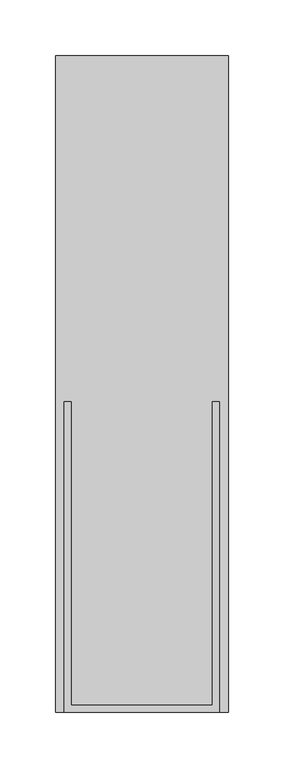
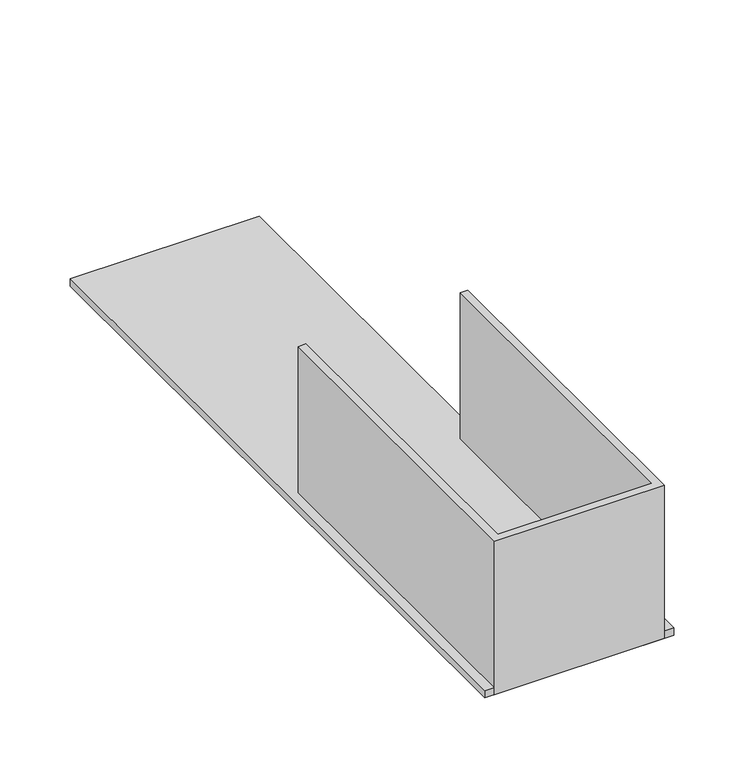
"""IFC4 building model written with IfcOpenShell, lengths in millimetres: fastener geometry, SIMPSON -THGBV - Truss Girder Hanger : SIMPSON -THGBV5.50/11 - HDG."""

import ifcopenshell
import ifcopenshell.guid

model = None  # the IFC model being written
_history = None  # IfcOwnerHistory: only IFC2X3 demands one
_inside = {}  # id of a spatial element -> (the spatial element, [elements in it])
_under = {}  # id of a project, library or spatial element -> (it, [spatial elements below it])
_declared = {}  # id of a project -> (the project, [libraries it declares])
_typed = {}  # id of a type object -> (the type object, [elements of that type])
_made_of = {}  # id of a material, layer set ... -> (it, [elements and type objects made of it])


def new_model(schema):
    """Start an empty IFC model of exactly this schema.

    Asked for "IFC4X3", IfcOpenShell would pick the latest addendum, in which some entities
    have other attributes; the version numbers below select the first issue.
    IFC2X3 requires an IfcOwnerHistory on every rooted entity: one is made here for all.
    """
    global model, _history
    if schema == "IFC4X3":
        model = ifcopenshell.file(schema_version=(4, 3, 0, 0))
    else:
        model = ifcopenshell.file(schema=schema)
    _inside.clear()
    _under.clear()
    _declared.clear()
    _typed.clear()
    _made_of.clear()
    _history = None
    if model.schema == "IFC2X3":
        org = make("IfcOrganization", Name="unknown")
        user = make(
            "IfcPersonAndOrganization",
            ThePerson=make("IfcPerson", FamilyName="unknown"),
            TheOrganization=org,
        )
        app = make(
            "IfcApplication",
            ApplicationDeveloper=org,
            Version="unknown",
            ApplicationFullName="unknown",
            ApplicationIdentifier="unknown",
        )
        _history = make(
            "IfcOwnerHistory",
            OwningUser=user,
            OwningApplication=app,
            ChangeAction="ADDED",
            CreationDate=0,
        )
    return model


def make(cls, **values):
    """One entity of the class cls with the attributes given. An attribute that is None is left unset."""
    return model.create_entity(
        cls, **{name: value for name, value in values.items() if value is not None}
    )


def rooted(cls, **values):
    """An entity with a GlobalId (a new one), such as an element, a storey or a relation."""
    return make(cls, GlobalId=ifcopenshell.guid.new(), OwnerHistory=_history, **values)


def si_unit(unit_type, name, prefix=None):
    """IfcSIUnit, for example si_unit("LENGTHUNIT", "METRE", prefix="MILLI")."""
    return make("IfcSIUnit", UnitType=unit_type, Prefix=prefix, Name=name)


def assignment(units):
    """IfcUnitAssignment: the units of a project."""
    return None if units is None else make("IfcUnitAssignment", Units=units)


def point(xyz):
    """IfcCartesianPoint."""
    return None if xyz is None else make("IfcCartesianPoint", Coordinates=xyz)


def direction(xyz):
    """IfcDirection."""
    return None if xyz is None else make("IfcDirection", DirectionRatios=xyz)


def frame(location, z_axis=None, x_axis=None):
    """IfcAxis2Placement3D, a coordinate frame: its origin and axes. An axis left out is left unset."""
    return make(
        "IfcAxis2Placement3D",
        Location=point(location),
        Axis=direction(z_axis),
        RefDirection=direction(x_axis),
    )


def origin():
    """The frame at (0, 0, 0) with its axes left unset."""
    return frame((0.0, 0.0, 0.0))


def origin_with_axes():
    """The frame at (0, 0, 0) with the z axis (0, 0, 1) and the x axis (1, 0, 0) written out."""
    return frame((0.0, 0.0, 0.0), z_axis=(0.0, 0.0, 1.0), x_axis=(1.0, 0.0, 0.0))


def place(relative_to, where):
    """IfcLocalPlacement: puts the frame where relative to a parent placement (None: the world)."""
    return make(
        "IfcLocalPlacement", PlacementRelTo=relative_to, RelativePlacement=where
    )


def context(
    kind, dimensions, precision=None, world=None, true_north=None, identifier=None
):
    """IfcGeometricRepresentationContext, for example the 3D "Model" context."""
    return make(
        "IfcGeometricRepresentationContext",
        ContextIdentifier=identifier,
        ContextType=kind,
        CoordinateSpaceDimension=dimensions,
        Precision=precision,
        WorldCoordinateSystem=world,
        TrueNorth=true_north,
    )


def project(units=None, contexts=None):
    """IfcProject with its units and contexts."""
    return rooted(
        "IfcProject",
        Name="project",
        RepresentationContexts=contexts,
        UnitsInContext=assignment(units),
    )


def spatial(cls, under=None, at=None, **own):
    """A site, building, storey or space (cls), placed at a placement, below another one or the project."""
    s = rooted(cls, ObjectPlacement=at, **own)
    if under is not None:
        _under.setdefault(under.id(), (under, []))[1].append(s)
    return s


def polyline(points):
    """IfcPolyline through the points."""
    return make("IfcPolyline", Points=[point(p) for p in points])


def outline(outer, holes=None, kind="AREA"):
    """IfcArbitraryClosedProfileDef: a profile drawn as a closed curve; with holes, ...WithVoids."""
    if holes is None:
        return make("IfcArbitraryClosedProfileDef", ProfileType=kind, OuterCurve=outer)
    return make(
        "IfcArbitraryProfileDefWithVoids",
        ProfileType=kind,
        OuterCurve=outer,
        InnerCurves=holes,
    )


def extrude(swept, where, along, depth):
    """IfcExtrudedAreaSolid: the profile swept, set in the frame where, extruded along a direction by depth."""
    return make(
        "IfcExtrudedAreaSolid",
        SweptArea=swept,
        Position=where,
        ExtrudedDirection=direction(along),
        Depth=depth,
    )


def shape(context_of_items, identifier, shape_type, items):
    """IfcShapeRepresentation: the items that make up one representation, for example the "Body"."""
    return make(
        "IfcShapeRepresentation",
        ContextOfItems=context_of_items,
        RepresentationIdentifier=identifier,
        RepresentationType=shape_type,
        Items=items,
    )


def source(mapping_origin, context_of_items, identifier, shape_type, items):
    """IfcRepresentationMap: a shape defined once, which mapped items show again and again."""
    return make(
        "IfcRepresentationMap",
        MappingOrigin=mapping_origin,
        MappedRepresentation=shape(context_of_items, identifier, shape_type, items),
    )


def transform(
    local_origin,
    x_axis=None,
    y_axis=None,
    z_axis=None,
    scale=None,
    scale2=None,
    scale3=None,
    uniform=True,
):
    """IfcCartesianTransformationOperator3D, or its non-uniform kind. x_axis, y_axis, z_axis: its Axis1, 2, 3."""
    if uniform:
        return make(
            "IfcCartesianTransformationOperator3D",
            Axis1=direction(x_axis),
            Axis2=direction(y_axis),
            LocalOrigin=point(local_origin),
            Scale=scale,
            Axis3=direction(z_axis),
        )
    return make(
        "IfcCartesianTransformationOperator3DnonUniform",
        Axis1=direction(x_axis),
        Axis2=direction(y_axis),
        LocalOrigin=point(local_origin),
        Scale=scale,
        Axis3=direction(z_axis),
        Scale2=scale2,
        Scale3=scale3,
    )


def mapped(mapping_source, mapping_target):
    """IfcMappedItem: shows the shape of a source again, moved by a transform."""
    return make(
        "IfcMappedItem", MappingSource=mapping_source, MappingTarget=mapping_target
    )


def made_of(thing, what):
    """Note that an element or type object is made of a material, layer set ...; save() writes the relation."""
    if what is not None:
        _made_of.setdefault(what.id(), (what, []))[1].append(thing)
    return thing


def element(
    cls,
    number,
    at=None,
    inside=None,
    cuts=None,
    type_object=None,
    material=None,
    context=None,
    identifier="Body",
    shape_type=None,
    held_by="IfcProductDefinitionShape",
    body=None,
    shapes=None,
    **own,
):
    """One element of the class cls, such as IfcWall. Its Tag is "e" and its number.

    at: its placement. inside: the storey or other place that contains it. cuts: it is an
    opening in that element (IfcRelVoidsElement). A single representation is given by context,
    identifier, shape_type and body (its items); several are given by shapes. held_by: the class
    of the entity that holds the representations. save() writes the other relations.
    """
    e = rooted(cls, Tag="e%d" % number, ObjectPlacement=at, **own)
    if body is not None:
        shapes = [shape(context, identifier, shape_type, body)]
    if shapes is not None:
        e.Representation = make(held_by, Representations=shapes)
    if inside is not None:
        _inside.setdefault(inside.id(), (inside, []))[1].append(e)
    if cuts is not None:
        rooted(
            "IfcRelVoidsElement", RelatingBuildingElement=cuts, RelatedOpeningElement=e
        )
    if type_object is not None:
        _typed.setdefault(type_object.id(), (type_object, []))[1].append(e)
    return made_of(e, material)


def aggregate(whole, parts):
    """IfcRelAggregates: a whole, such as a stair, and the parts it consists of."""
    return rooted("IfcRelAggregates", RelatingObject=whole, RelatedObjects=parts)


def save(model, path):
    """Write the relations noted so far, then the file.

    IfcRelAggregates (storeys below a building ...), IfcRelContainedInSpatialStructure (elements
    in a storey), IfcRelDefinesByType, IfcRelAssociatesMaterial and IfcRelDeclares: one each for
    every whole, place, type object, material and project.
    """
    for whole, parts in _under.values():
        aggregate(whole, parts)
    for where, things in _inside.values():
        rooted(
            "IfcRelContainedInSpatialStructure",
            RelatedElements=things,
            RelatingStructure=where,
        )
    for kind, things in _typed.values():
        rooted("IfcRelDefinesByType", RelatedObjects=things, RelatingType=kind)
    for what, things in _made_of.values():
        rooted("IfcRelAssociatesMaterial", RelatedObjects=things, RelatingMaterial=what)
    for by, libraries in _declared.values():
        rooted("IfcRelDeclares", RelatingContext=by, RelatedDefinitions=libraries)
    model.write(path)


def fastener_118951d1(model_context):
    return source(origin(), model_context, "Body", "SweptSolid", [
        extrude(outline(polyline([(-69.85, 0.0), (-69.85, 279.4), (-63.5, 279.4), (-63.5, 6.35), (63.5, 6.35), (63.5, 279.4), (69.85, 279.4), (69.85, 0.0), (-69.85, 0.0)])), origin_with_axes(), (0.0, 0.0, 1.0), 133.35),
        extrude(outline(polyline([(77.7875, 590.55), (77.7875, 0.0), (-77.7875, 0.0), (-77.7875, 590.55), (77.7875, 590.55)])), origin_with_axes(), (0.0, 0.0, 1.0), 6.35),
    ])


if __name__ == "__main__":
    model = new_model("IFC4")
    model_context = context("Model", 3, world=origin())
    ifc_project = project(units=[si_unit("LENGTHUNIT", "METRE", prefix="MILLI")], contexts=[model_context])
    site = spatial("IfcSite", under=ifc_project)
    building = spatial("IfcBuilding", under=site)
    placement = place(None, origin())
    fastener_shape = fastener_118951d1(model_context)
    element("IfcFastener", 1, ObjectType="SIMPSON -THGBV - Truss Girder Hanger : SIMPSON -THGBV5.50/11 - HDG", at=placement, inside=building, context=model_context, shape_type="MappedRepresentation", body=[
        mapped(fastener_shape, transform((0.0, 0.0, 0.0), x_axis=(1.0, 0.0, 0.0), y_axis=(0.0, 1.0, 0.0), z_axis=(0.0, 0.0, 1.0))),
    ])
    save(model, "model.ifc")

# Revit data of these elements
# Type "SIMPSON -THGBV - Truss Girder Hanger : SIMPSON -THGBV5.50/11 - HDG"
#   URL = "http://embed.widencdn.net/pdf/plus/ssttoolbox/iecrxc4cbv/C-C-2017-p254-255.pdf"
#   W = 0' - 5 1/2"
#   H = 0' - 11"
#   Default Elevation = 4' - 0"
